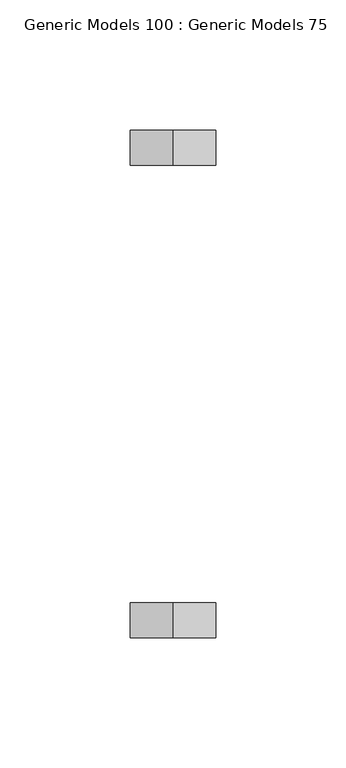
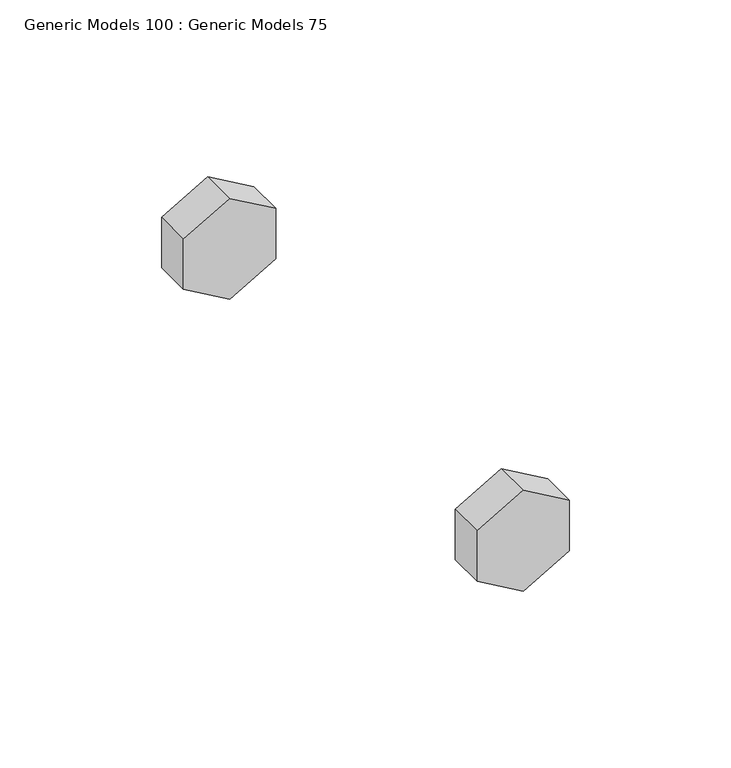
"""IFC4 building model written with IfcOpenShell, lengths in millimetres: proxy geometry, Generic Models 100 : Generic Models 75."""

import ifcopenshell
import ifcopenshell.guid

model = None  # the IFC model being written
_history = None  # IfcOwnerHistory: only IFC2X3 demands one
_inside = {}  # id of a spatial element -> (the spatial element, [elements in it])
_under = {}  # id of a project, library or spatial element -> (it, [spatial elements below it])
_declared = {}  # id of a project -> (the project, [libraries it declares])
_typed = {}  # id of a type object -> (the type object, [elements of that type])
_made_of = {}  # id of a material, layer set ... -> (it, [elements and type objects made of it])


def new_model(schema):
    """Start an empty IFC model of exactly this schema.

    Asked for "IFC4X3", IfcOpenShell would pick the latest addendum, in which some entities
    have other attributes; the version numbers below select the first issue.
    IFC2X3 requires an IfcOwnerHistory on every rooted entity: one is made here for all.
    """
    global model, _history
    if schema == "IFC4X3":
        model = ifcopenshell.file(schema_version=(4, 3, 0, 0))
    else:
        model = ifcopenshell.file(schema=schema)
    _inside.clear()
    _under.clear()
    _declared.clear()
    _typed.clear()
    _made_of.clear()
    _history = None
    if model.schema == "IFC2X3":
        org = make("IfcOrganization", Name="unknown")
        user = make(
            "IfcPersonAndOrganization",
            ThePerson=make("IfcPerson", FamilyName="unknown"),
            TheOrganization=org,
        )
        app = make(
            "IfcApplication",
            ApplicationDeveloper=org,
            Version="unknown",
            ApplicationFullName="unknown",
            ApplicationIdentifier="unknown",
        )
        _history = make(
            "IfcOwnerHistory",
            OwningUser=user,
            OwningApplication=app,
            ChangeAction="ADDED",
            CreationDate=0,
        )
    return model


def make(cls, **values):
    """One entity of the class cls with the attributes given. An attribute that is None is left unset."""
    return model.create_entity(
        cls, **{name: value for name, value in values.items() if value is not None}
    )


def rooted(cls, **values):
    """An entity with a GlobalId (a new one), such as an element, a storey or a relation."""
    return make(cls, GlobalId=ifcopenshell.guid.new(), OwnerHistory=_history, **values)


def si_unit(unit_type, name, prefix=None):
    """IfcSIUnit, for example si_unit("LENGTHUNIT", "METRE", prefix="MILLI")."""
    return make("IfcSIUnit", UnitType=unit_type, Prefix=prefix, Name=name)


def assignment(units):
    """IfcUnitAssignment: the units of a project."""
    return None if units is None else make("IfcUnitAssignment", Units=units)


def point(xyz):
    """IfcCartesianPoint."""
    return None if xyz is None else make("IfcCartesianPoint", Coordinates=xyz)


def direction(xyz):
    """IfcDirection."""
    return None if xyz is None else make("IfcDirection", DirectionRatios=xyz)


def frame(location, z_axis=None, x_axis=None):
    """IfcAxis2Placement3D, a coordinate frame: its origin and axes. An axis left out is left unset."""
    return make(
        "IfcAxis2Placement3D",
        Location=point(location),
        Axis=direction(z_axis),
        RefDirection=direction(x_axis),
    )


def origin():
    """The frame at (0, 0, 0) with its axes left unset."""
    return frame((0.0, 0.0, 0.0))


def place(relative_to, where):
    """IfcLocalPlacement: puts the frame where relative to a parent placement (None: the world)."""
    return make(
        "IfcLocalPlacement", PlacementRelTo=relative_to, RelativePlacement=where
    )


def context(
    kind, dimensions, precision=None, world=None, true_north=None, identifier=None
):
    """IfcGeometricRepresentationContext, for example the 3D "Model" context."""
    return make(
        "IfcGeometricRepresentationContext",
        ContextIdentifier=identifier,
        ContextType=kind,
        CoordinateSpaceDimension=dimensions,
        Precision=precision,
        WorldCoordinateSystem=world,
        TrueNorth=true_north,
    )


def project(units=None, contexts=None):
    """IfcProject with its units and contexts."""
    return rooted(
        "IfcProject",
        Name="project",
        RepresentationContexts=contexts,
        UnitsInContext=assignment(units),
    )


def spatial(cls, under=None, at=None, **own):
    """A site, building, storey or space (cls), placed at a placement, below another one or the project."""
    s = rooted(cls, ObjectPlacement=at, **own)
    if under is not None:
        _under.setdefault(under.id(), (under, []))[1].append(s)
    return s


def polyline(points):
    """IfcPolyline through the points."""
    return make("IfcPolyline", Points=[point(p) for p in points])


def outline(outer, holes=None, kind="AREA"):
    """IfcArbitraryClosedProfileDef: a profile drawn as a closed curve; with holes, ...WithVoids."""
    if holes is None:
        return make("IfcArbitraryClosedProfileDef", ProfileType=kind, OuterCurve=outer)
    return make(
        "IfcArbitraryProfileDefWithVoids",
        ProfileType=kind,
        OuterCurve=outer,
        InnerCurves=holes,
    )


def extrude(swept, where, along, depth):
    """IfcExtrudedAreaSolid: the profile swept, set in the frame where, extruded along a direction by depth."""
    return make(
        "IfcExtrudedAreaSolid",
        SweptArea=swept,
        Position=where,
        ExtrudedDirection=direction(along),
        Depth=depth,
    )


def shape(context_of_items, identifier, shape_type, items):
    """IfcShapeRepresentation: the items that make up one representation, for example the "Body"."""
    return make(
        "IfcShapeRepresentation",
        ContextOfItems=context_of_items,
        RepresentationIdentifier=identifier,
        RepresentationType=shape_type,
        Items=items,
    )


def source(mapping_origin, context_of_items, identifier, shape_type, items):
    """IfcRepresentationMap: a shape defined once, which mapped items show again and again."""
    return make(
        "IfcRepresentationMap",
        MappingOrigin=mapping_origin,
        MappedRepresentation=shape(context_of_items, identifier, shape_type, items),
    )


def transform(
    local_origin,
    x_axis=None,
    y_axis=None,
    z_axis=None,
    scale=None,
    scale2=None,
    scale3=None,
    uniform=True,
):
    """IfcCartesianTransformationOperator3D, or its non-uniform kind. x_axis, y_axis, z_axis: its Axis1, 2, 3."""
    if uniform:
        return make(
            "IfcCartesianTransformationOperator3D",
            Axis1=direction(x_axis),
            Axis2=direction(y_axis),
            LocalOrigin=point(local_origin),
            Scale=scale,
            Axis3=direction(z_axis),
        )
    return make(
        "IfcCartesianTransformationOperator3DnonUniform",
        Axis1=direction(x_axis),
        Axis2=direction(y_axis),
        LocalOrigin=point(local_origin),
        Scale=scale,
        Axis3=direction(z_axis),
        Scale2=scale2,
        Scale3=scale3,
    )


def mapped(mapping_source, mapping_target):
    """IfcMappedItem: shows the shape of a source again, moved by a transform."""
    return make(
        "IfcMappedItem", MappingSource=mapping_source, MappingTarget=mapping_target
    )


def made_of(thing, what):
    """Note that an element or type object is made of a material, layer set ...; save() writes the relation."""
    if what is not None:
        _made_of.setdefault(what.id(), (what, []))[1].append(thing)
    return thing


def element(
    cls,
    number,
    at=None,
    inside=None,
    cuts=None,
    type_object=None,
    material=None,
    context=None,
    identifier="Body",
    shape_type=None,
    held_by="IfcProductDefinitionShape",
    body=None,
    shapes=None,
    **own,
):
    """One element of the class cls, such as IfcWall. Its Tag is "e" and its number.

    at: its placement. inside: the storey or other place that contains it. cuts: it is an
    opening in that element (IfcRelVoidsElement). A single representation is given by context,
    identifier, shape_type and body (its items); several are given by shapes. held_by: the class
    of the entity that holds the representations. save() writes the other relations.
    """
    e = rooted(cls, Tag="e%d" % number, ObjectPlacement=at, **own)
    if body is not None:
        shapes = [shape(context, identifier, shape_type, body)]
    if shapes is not None:
        e.Representation = make(held_by, Representations=shapes)
    if inside is not None:
        _inside.setdefault(inside.id(), (inside, []))[1].append(e)
    if cuts is not None:
        rooted(
            "IfcRelVoidsElement", RelatingBuildingElement=cuts, RelatedOpeningElement=e
        )
    if type_object is not None:
        _typed.setdefault(type_object.id(), (type_object, []))[1].append(e)
    return made_of(e, material)


def aggregate(whole, parts):
    """IfcRelAggregates: a whole, such as a stair, and the parts it consists of."""
    return rooted("IfcRelAggregates", RelatingObject=whole, RelatedObjects=parts)


def save(model, path):
    """Write the relations noted so far, then the file.

    IfcRelAggregates (storeys below a building ...), IfcRelContainedInSpatialStructure (elements
    in a storey), IfcRelDefinesByType, IfcRelAssociatesMaterial and IfcRelDeclares: one each for
    every whole, place, type object, material and project.
    """
    for whole, parts in _under.values():
        aggregate(whole, parts)
    for where, things in _inside.values():
        rooted(
            "IfcRelContainedInSpatialStructure",
            RelatedElements=things,
            RelatingStructure=where,
        )
    for kind, things in _typed.values():
        rooted("IfcRelDefinesByType", RelatedObjects=things, RelatingType=kind)
    for what, things in _made_of.values():
        rooted("IfcRelAssociatesMaterial", RelatedObjects=things, RelatingMaterial=what)
    for by, libraries in _declared.values():
        rooted("IfcRelDeclares", RelatingContext=by, RelatedDefinitions=libraries)
    model.write(path)


def generic_models_100_generic_models_75_5ab5e8ab(model_context):
    return source(origin(), model_context, "Body", "SweptSolid", [
        extrude(outline(polyline([(266616.6501684, 31991.9073871), (266635.7001684, 31991.9073871), (266645.2251684, 31975.4096032), (266635.7001684, 31958.9118192), (266616.6501684, 31958.9118192), (266607.1251684, 31975.4096032), (266616.6501684, 31991.9073871)])), frame((0.0, 35373.9582942, 0.0), z_axis=(0.0, 1.0, 0.0), x_axis=(0.0, 0.0, 1.0)), (0.0, 0.0, 1.0), 13.49375),
        extrude(outline(polyline([(266616.6501684, 31991.9073871), (266635.7001684, 31991.9073871), (266645.2251684, 31975.4096032), (266635.7001684, 31958.9118192), (266616.6501684, 31958.9118192), (266607.1251684, 31975.4096032), (266616.6501684, 31991.9073871)])), frame((0.0, 35192.1895442, 0.0), z_axis=(0.0, 1.0, 0.0), x_axis=(0.0, 0.0, 1.0)), (0.0, 0.0, 1.0), 13.49375),
    ])


if __name__ == "__main__":
    model = new_model("IFC4")
    model_context = context("Model", 3, world=origin())
    ifc_project = project(units=[si_unit("LENGTHUNIT", "METRE", prefix="MILLI")], contexts=[model_context])
    site = spatial("IfcSite", under=ifc_project)
    building = spatial("IfcBuilding", under=site)
    placement = place(None, origin())
    generic_models_100_generic_models_75_shape = generic_models_100_generic_models_75_5ab5e8ab(model_context)
    element("IfcBuildingElementProxy", 1, Name="Generic Models 100 : Generic Models 75", ObjectType="Generic Models 100 : Generic Models 75", at=placement, inside=building, context=model_context, shape_type="MappedRepresentation", body=[
        mapped(generic_models_100_generic_models_75_shape, transform((0.0, 0.0, 0.0), x_axis=(1.0, 0.0, 0.0), y_axis=(0.0, 1.0, 0.0), z_axis=(0.0, 0.0, 1.0))),
    ])
    save(model, "model.ifc")
